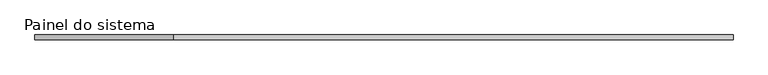
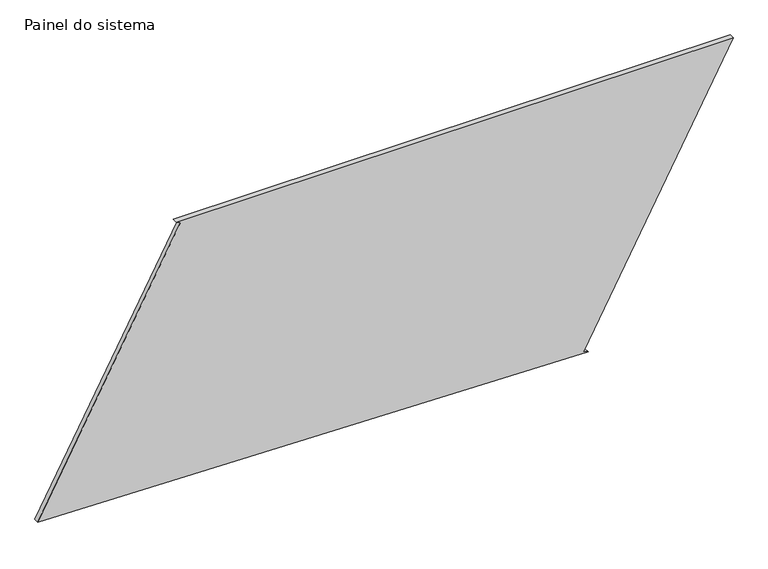
"""IFC4 building model written with IfcOpenShell, lengths in millimetres: plate geometry, Painel do sistema : Envidraçado."""

from ifc_helpers import new_model, si_unit, frame, origin, place, context, project, spatial, polyline, outline, extrude, source, transform, mapped, element, save


def painel_do_sistema_2b943041(model_context):
    return source(origin(), model_context, "Body", "SweptSolid", [
        extrude(outline(polyline([(0.0, 1051.1216831), (11.7958757, 1029.0795117), (1459.1635925, 1803.6388489), (1459.1635925, -1085.8552245), (1447.3677169, -1063.8130532), (64.9042677, -1803.6388489), (0.0, 1051.1216831)])), frame((0.0, 24.5, 0.0), z_axis=(0.0, 1.0, 0.0), x_axis=(0.0, 0.0, 1.0)), (0.0, 0.0, 1.0), 25.0),
    ])


if __name__ == "__main__":
    model = new_model("IFC4")
    model_context = context("Model", 3, world=origin())
    ifc_project = project(units=[si_unit("LENGTHUNIT", "METRE", prefix="MILLI")], contexts=[model_context])
    site = spatial("IfcSite", under=ifc_project)
    building = spatial("IfcBuilding", under=site)
    placement = place(None, origin())
    painel_do_sistema_shape = painel_do_sistema_2b943041(model_context)
    element("IfcPlate", 1, ObjectType="Painel do sistema : Envidraçado", at=placement, inside=building, context=model_context, shape_type="MappedRepresentation", body=[
        mapped(painel_do_sistema_shape, transform((0.0, 0.0, 0.0), x_axis=(1.0, 0.0, 0.0), y_axis=(0.0, 1.0, 0.0), z_axis=(0.0, 0.0, 1.0))),
    ])
    save(model, "model.ifc")

# Revit data of these elements
# Type "Painel do sistema : Envidraçado"
#   Construction Type Id = "GSP4R"
#   Analytic Construction = "Vidraça única Pilkington 1/8 pol"
#   Visual Light Transmittance = 0.9
#   Solar Heat Gain Coefficient = 0.86
#   Heat Transfer Coefficient (U) = 6.7069 W/(m²·K)
# Element 1 (IfcPlate, "Painel do sistema : Envidraçado")
#   Materials on its faces: "Vidro"
# Materials
#   "Vidro": class "Vidro", colour RGB 0 128 192, transparency 0.9, Description = "Vidro de sílica", Cost = 0
